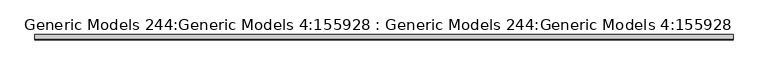
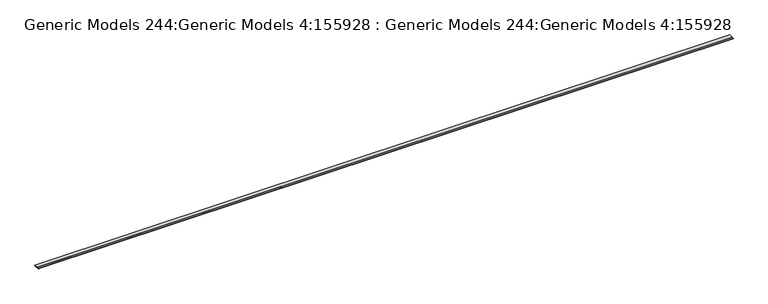
"""IFC4 building model written with IfcOpenShell, lengths in millimetres: proxy geometry, Generic Models 244:Generic Models 4:155928 : Generic Models 244:Generic Models 4:155928."""

from ifc_helpers import new_model, si_unit, frame, origin, place, context, project, spatial, polyline, outline, extrude, source, transform, mapped, element, save


def generic_models_244_generic_models_4_155928_generic_models_ecc88eef(model_context):
    return source(origin(), model_context, "Body", "SweptSolid", [
        extrude(outline(polyline([(12032.1928662, 3067.05), (12144.1675942, 3067.05), (12144.1675942, 3046.095), (12121.7244102, 3046.095), (12121.7244102, 3044.825), (11998.8426662, 3044.825), (11998.8426662, 3047.8274564), (11997.5726662, 3047.8274564), (11997.5726662, 3046.095), (11995.3628662, 3046.095), (11995.3628662, 3065.78), (12032.1928662, 3065.78), (12032.1928662, 3067.05)])), frame((-10407.6290248, 0.0, 0.0), z_axis=(1.0, 0.0, 0.0), x_axis=(0.0, 1.0, 0.0)), (0.0, 0.0, 1.0), 18643.6),
    ])


if __name__ == "__main__":
    model = new_model("IFC4")
    model_context = context("Model", 3, world=origin())
    ifc_project = project(units=[si_unit("LENGTHUNIT", "METRE", prefix="MILLI")], contexts=[model_context])
    site = spatial("IfcSite", under=ifc_project)
    building = spatial("IfcBuilding", under=site)
    placement = place(None, origin())
    generic_models_244_generic_models_4_155928_generic_models_shape = generic_models_244_generic_models_4_155928_generic_models_ecc88eef(model_context)
    element("IfcBuildingElementProxy", 1, Name="Generic Models 244:Generic Models 4:155928 : Generic Models 244:Generic Models 4:155928", ObjectType="Generic Models 244:Generic Models 4:155928 : Generic Models 244:Generic Models 4:155928", at=placement, inside=building, context=model_context, shape_type="MappedRepresentation", body=[
        mapped(generic_models_244_generic_models_4_155928_generic_models_shape, transform((0.0, 0.0, 0.0), x_axis=(1.0, 0.0, 0.0), y_axis=(0.0, 1.0, 0.0), z_axis=(0.0, 0.0, 1.0))),
    ])
    save(model, "model.ifc")

# Revit data of these elements
# Type "Generic Models 244:Generic Models 4:155928 : Generic Models 244:Generic Models 4:155928"
#   NameOverride = "Generic Models 244:Generic Models 4:155928"
#   ObjectTypeOverride = "Generic Models 244:Generic Models 4"
#   Reference = "Generic Models 4"
#   Category = "Generic Models"
#   Tag = "155928"
# Element 1 (IfcBuildingElementProxy, "Generic Models 244:Generic Models 4:155928 : Generic Models 244:Generic Models 4:155928")
#   Materials on its faces: "_7/8\" SMOOTH TROWEL EXTERIOR STUCCO (COLOR PER OWNER) 770"
# Materials
#   "_7/8\" SMOOTH TROWEL EXTERIOR STUCCO (COLOR PER OWNER) 770": class "Unassigned", colour RGB 233 233 233, transparency 0
